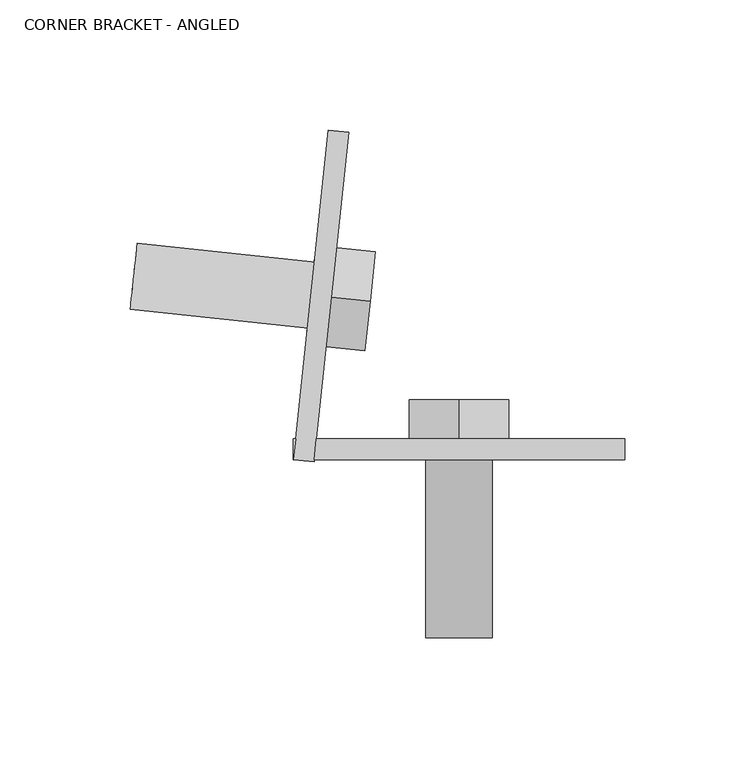
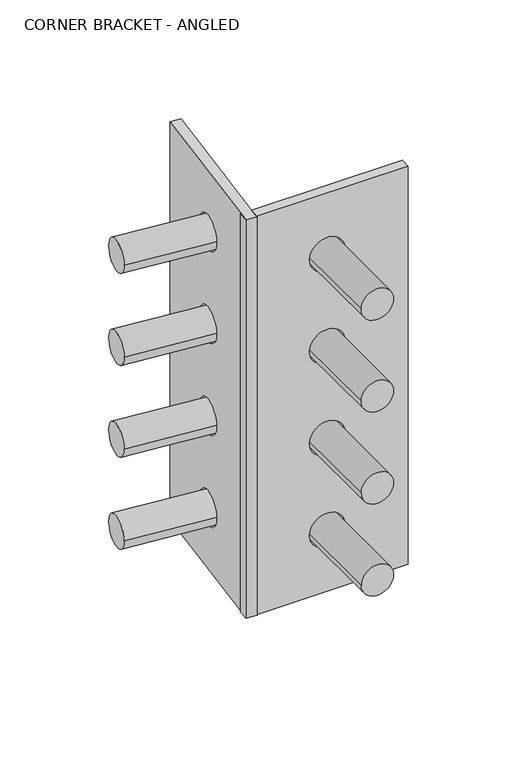
"""IFC4 building model written with IfcOpenShell, lengths in millimetres: fastener geometry, CORNER BRACKET - ANGLED."""

from ifc_helpers import new_model, si_unit, point, frame, frame_2d, origin, place, context, project, spatial, polyline, circle_curve, trimmed, segment, composite_curve, outline, extrude, faceted_brep, source, transform, mapped, element, save
from ifc_brep_helpers import plane_surface, revolved_surface, advanced_brep


def corner_bracket_angled_f47ab821(model_context):
    return source(origin(), model_context, "Body", "SolidModel", [
        advanced_brep(
        [(49.609375, 7.9375, 203.2), (77.390625, 7.9375, 203.2), (77.390625, 0.0, 203.2), (49.609375, 0.0, 203.2), (77.390625, 7.9375, 279.4), (49.609375, 7.9375, 279.4), (49.609375, 0.0, 279.4), (77.390625, 0.0, 279.4), (127.0, 0.0, 0.0), (127.0, 7.9375, 0.0), (127.0, 7.9375, 330.2), (127.0, 0.0, 330.2), (77.390625, 0.0, 127.0), (49.609375, 0.0, 127.0), (49.609375, 7.9375, 127.0), (77.390625, 7.9375, 127.0), (77.390625, 0.0, 50.8), (49.609375, 0.0, 50.8), (49.609375, 7.9375, 50.8), (77.390625, 7.9375, 50.8), (7.981222, 0.0, 330.2), (7.981222, 0.0, 0.0), (8.8154868, 7.9375, 0.0), (8.8154868, 7.9375, 330.2)],
        [
            (0, 1, circle_curve(frame((63.5, 7.9375, 203.2), z_axis=(0.0, 1.0, 0.0), x_axis=(-1.0000000000000002, 0.0, 0.0)), 13.890625)),
            (1, 2),
            (2, 3, circle_curve(frame((63.5, 0.0, 203.2), z_axis=(0.0, -1.0, 0.0), x_axis=(-1.0000000000000002, 0.0, 0.0)), 13.890625)),
            (3, 0),
            (4, 5, circle_curve(frame((63.5, 7.9375, 279.4), z_axis=(0.0, 1.0, 0.0), x_axis=(-1.0000000000000002, 0.0, 0.0)), 13.890625)),
            (5, 6),
            (6, 7, circle_curve(frame((63.5, 0.0, 279.4), z_axis=(0.0, -1.0, 0.0), x_axis=(-1.0000000000000002, 0.0, 0.0)), 13.890625)),
            (7, 4),
            (8, 9),
            (9, 10),
            (10, 11),
            (11, 8),
            (5, 4, circle_curve(frame((63.5, 7.9375, 279.4), z_axis=(0.0, 1.0, 0.0), x_axis=(-1.0000000000000002, 0.0, 0.0)), 13.890625)),
            (7, 6, circle_curve(frame((63.5, 0.0, 279.4), z_axis=(0.0, -1.0, 0.0), x_axis=(-1.0000000000000002, 0.0, 0.0)), 13.890625)),
            (12, 13, circle_curve(frame((63.5, 0.0, 127.0), z_axis=(0.0, -1.0, 0.0), x_axis=(-1.0000000000000002, 0.0, 0.0)), 13.890625)),
            (13, 14),
            (14, 15, circle_curve(frame((63.5, 7.9375, 127.0), z_axis=(0.0, 1.0, 0.0), x_axis=(-1.0000000000000002, 0.0, 0.0)), 13.890625)),
            (15, 12),
            (16, 17, circle_curve(frame((63.5, 0.0, 50.8), z_axis=(0.0, -1.0, 0.0), x_axis=(-1.0000000000000002, 0.0, 0.0)), 13.890625)),
            (17, 18),
            (18, 19, circle_curve(frame((63.5, 7.9375, 50.8), z_axis=(0.0, 1.0, 0.0), x_axis=(-1.0000000000000002, 0.0, 0.0)), 13.890625)),
            (19, 16),
            (11, 20),
            (20, 21),
            (21, 8),
            (2, 3, circle_curve(frame((63.5, 0.0, 203.2), z_axis=(0.0, 1.0, 0.0), x_axis=(-1.0000000000000002, 0.0, 0.0)), 13.890625)),
            (12, 13, circle_curve(frame((63.5, 0.0, 127.0), z_axis=(0.0, 1.0, 0.0), x_axis=(-1.0000000000000002, 0.0, 0.0)), 13.890625)),
            (16, 17, circle_curve(frame((63.5, 0.0, 50.8), z_axis=(0.0, 1.0, 0.0), x_axis=(-1.0000000000000002, 0.0, 0.0)), 13.890625)),
            (21, 22),
            (22, 9),
            (1, 0, circle_curve(frame((63.5, 7.9375, 203.2), z_axis=(0.0, 1.0, 0.0), x_axis=(-1.0000000000000002, 0.0, 0.0)), 13.890625)),
            (15, 14, circle_curve(frame((63.5, 7.9375, 127.0), z_axis=(0.0, 1.0, 0.0), x_axis=(-1.0000000000000002, 0.0, 0.0)), 13.890625)),
            (19, 18, circle_curve(frame((63.5, 7.9375, 50.8), z_axis=(0.0, 1.0, 0.0), x_axis=(-1.0000000000000002, 0.0, 0.0)), 13.890625)),
            (23, 22),
            (20, 23),
            (23, 10),
        ],
        [
            revolved_surface(polyline([(49.609375, 7.937500000000007, 203.2), (49.609375, 0.0, 203.2)]), (63.5, 0.0, 203.2), (0.0, 1.0000000000000004, 0.0)),
            revolved_surface(polyline([(49.609375, 7.937500000000007, 279.4), (49.609375, 0.0, 279.4)]), (63.5, 0.0, 279.4), (0.0, 1.0000000000000004, 0.0)),
            plane_surface(frame((127.0, 7.9375, 330.2), z_axis=(1.0, 0.0, 0.0), x_axis=(0.0, -1.0, 0.0))),
            revolved_surface(polyline([(49.609375, 7.937500000000007, 127.0), (49.609375, 0.0, 127.0)]), (63.5, 0.0, 127.0), (0.0, 1.0000000000000004, 0.0)),
            revolved_surface(polyline([(49.609375, 7.937500000000007, 50.8), (49.609375, 0.0, 50.8)]), (63.5, 0.0, 50.8), (0.0, 1.0000000000000004, 0.0)),
            plane_surface(frame((127.0, 0.0, 330.2), z_axis=(0.0, -1.0, 0.0), x_axis=(-1.0, 0.0, 0.0))),
            plane_surface(frame((127.0, 7.9375, 0.0), z_axis=(0.0, 0.0, -1.0), x_axis=(0.0, -1.0, 0.0))),
            plane_surface(frame((21.1691324, 125.474586, 330.2), z_axis=(-0.9945218953682732, 0.10452846326765532, 0.0), x_axis=(0.10452846326765532, 0.9945218953682732, 0.0))),
            plane_surface(frame((127.0, 7.9375, 330.2), z_axis=(0.0, 1.0, 0.0), x_axis=(1.0, 0.0, 0.0))),
            plane_surface(frame((0.0, 7.9375, 330.2), z_axis=(0.0, 0.0, 1.0), x_axis=(0.0, -1.0, 0.0))),
        ],
        [
            (0, [[1, 2, 3, 4]]),
            (1, [[5, 6, 7, 8]]),
            (2, [[9, 10, 11, 12]]),
            (1, [[13, -8, 14, -6]]),
            (3, [[15, 16, 17, 18]]),
            (4, [[19, 20, 21, 22]]),
            (5, [[-12, 23, 24, 25], [-7, -14], [26, -3], [-15, 27], [28, -19]]),
            (6, [[-9, -25, 29, 30]]),
            (0, [[31, -4, -26, -2]]),
            (3, [[32, -16, -27, -18]]),
            (4, [[33, -20, -28, -22]]),
            (7, [[34, -29, -24, 35]]),
            (8, [[-10, -30, -34, 36], [-5, -13], [-32, -17], [-31, -1], [-33, -21]]),
            (9, [[-11, -36, -35, -23]]),
        ],
    ),
        faceted_brep([(0.0, 7.9375, 0.0), (0.0, 7.9375, 330.2), (0.8342649, 7.9375, 330.2), (0.8342649, 7.9375, 0.0), (0.0, 0.0, 330.2), (0.0, 0.0, 0.0)], [[[0, 1, 2, 3]], [[1, 4, 2]], [[1, 0, 5, 4]], [[3, 2, 4, 5]], [[5, 0, 3]]]),
        extrude(outline(polyline([(290.3985226, 82.55), (301.3970453, 63.5), (290.3985226, 44.45), (268.4014774, 44.45), (257.4029547, 63.5), (268.4014774, 82.55), (290.3985226, 82.55)])), frame((0.0, 7.9375, 0.0), z_axis=(0.0, 1.0, 0.0), x_axis=(0.0, 0.0, 1.0)), (0.0, 0.0, 1.0), 14.9820312),
        extrude(outline(composite_curve([segment(trimmed(circle_curve(frame_2d((279.4, 63.5)), 12.7), [point((279.4, 76.2))], [point((279.4, 50.8))], False, "CARTESIAN"), True, "CONTINUOUS"), segment(trimmed(circle_curve(frame_2d((279.4, 63.5)), 12.7), [point((279.4, 50.8))], [point((279.4, 76.2))], False, "CARTESIAN"), True, "CONTINUOUS")], self_intersect=False)), frame((0.0, -68.2625, 0.0), z_axis=(0.0, 1.0, 0.0), x_axis=(0.0, 0.0, 1.0)), (0.0, 0.0, 1.0), 76.2),
        extrude(outline(polyline([(214.1985226, 82.55), (225.1970453, 63.5), (214.1985226, 44.45), (192.2014774, 44.45), (181.2029547, 63.5), (192.2014774, 82.55), (214.1985226, 82.55)])), frame((0.0, 7.9375, 0.0), z_axis=(0.0, 1.0, 0.0), x_axis=(0.0, 0.0, 1.0)), (0.0, 0.0, 1.0), 14.9820312),
        extrude(outline(composite_curve([segment(trimmed(circle_curve(frame_2d((203.2, 63.5)), 12.7), [point((203.2, 76.2))], [point((203.2, 50.8))], False, "CARTESIAN"), True, "CONTINUOUS"), segment(trimmed(circle_curve(frame_2d((203.2, 63.5)), 12.7), [point((203.2, 50.8))], [point((203.2, 76.2))], False, "CARTESIAN"), True, "CONTINUOUS")], self_intersect=False)), frame((0.0, -68.2625, 0.0), z_axis=(0.0, 1.0, 0.0), x_axis=(0.0, 0.0, 1.0)), (0.0, 0.0, 1.0), 76.2),
        extrude(outline(polyline([(290.3985226, 82.55), (301.3970453, 63.5), (290.3985226, 44.45), (268.4014774, 44.45), (257.4029547, 63.5), (268.4014774, 82.55), (290.3985226, 82.55)])), frame((0.0, 7.9375, 0.0), z_axis=(0.0, 1.0, 0.0), x_axis=(0.0, 0.0, 1.0)), (0.0, 0.0, 1.0), 14.9820312),
        extrude(outline(composite_curve([segment(trimmed(circle_curve(frame_2d((279.4, 63.5)), 12.7), [point((279.4, 76.2))], [point((279.4, 50.8))], False, "CARTESIAN"), True, "CONTINUOUS"), segment(trimmed(circle_curve(frame_2d((279.4, 63.5)), 12.7), [point((279.4, 50.8))], [point((279.4, 76.2))], False, "CARTESIAN"), True, "CONTINUOUS")], self_intersect=False)), frame((0.0, -68.2625, 0.0), z_axis=(0.0, 1.0, 0.0), x_axis=(0.0, 0.0, 1.0)), (0.0, 0.0, 1.0), 76.2),
        extrude(outline(polyline([(137.9985226, 82.55), (148.9970453, 63.5), (137.9985226, 44.45), (116.0014774, 44.45), (105.0029547, 63.5), (116.0014774, 82.55), (137.9985226, 82.55)])), frame((0.0, 7.9375, 0.0), z_axis=(0.0, 1.0, 0.0), x_axis=(0.0, 0.0, 1.0)), (0.0, 0.0, 1.0), 14.9820312),
        extrude(outline(composite_curve([segment(trimmed(circle_curve(frame_2d((127.0, 63.5)), 12.7), [point((127.0, 76.2))], [point((127.0, 50.8))], False, "CARTESIAN"), True, "CONTINUOUS"), segment(trimmed(circle_curve(frame_2d((127.0, 63.5)), 12.7), [point((127.0, 50.8))], [point((127.0, 76.2))], False, "CARTESIAN"), True, "CONTINUOUS")], self_intersect=False)), frame((0.0, -68.2625, 0.0), z_axis=(0.0, 1.0, 0.0), x_axis=(0.0, 0.0, 1.0)), (0.0, 0.0, 1.0), 76.2),
        extrude(outline(polyline([(61.7985226, 82.55), (72.7970453, 63.5), (61.7985226, 44.45), (39.8014774, 44.45), (28.8029547, 63.5), (39.8014774, 82.55), (61.7985226, 82.55)])), frame((0.0, 7.9375, 0.0), z_axis=(0.0, 1.0, 0.0), x_axis=(0.0, 0.0, 1.0)), (0.0, 0.0, 1.0), 14.9820312),
        extrude(outline(composite_curve([segment(trimmed(circle_curve(frame_2d((50.8, 63.5)), 12.7), [point((50.8, 76.2))], [point((50.8, 50.8))], False, "CARTESIAN"), True, "CONTINUOUS"), segment(trimmed(circle_curve(frame_2d((50.8, 63.5)), 12.7), [point((50.8, 50.8))], [point((50.8, 76.2))], False, "CARTESIAN"), True, "CONTINUOUS")], self_intersect=False)), frame((0.0, -68.2625, 0.0), z_axis=(0.0, 1.0, 0.0), x_axis=(0.0, 0.0, 1.0)), (0.0, 0.0, 1.0), 76.2),
        advanced_brep(
        [(15.9835406, 76.1369764, 203.2), (13.0796093, 48.507915, 203.2), (5.1855917, 49.3376097, 203.2), (8.0895231, 76.9666711, 203.2), (8.0895231, 76.9666711, 279.4), (5.1855917, 49.3376097, 279.4), (13.0796093, 48.507915, 279.4), (15.9835406, 76.1369764, 279.4), (21.1691324, 125.474586, 0.0), (13.2751148, 126.3042807, 0.0), (13.2751148, 126.3042807, 330.2), (21.1691324, 125.474586, 330.2), (15.9835406, 76.1369764, 127.0), (13.0796093, 48.507915, 127.0), (5.1855917, 49.3376097, 127.0), (8.0895231, 76.9666711, 127.0), (15.9835406, 76.1369764, 50.8), (13.0796093, 48.507915, 50.8), (5.1855917, 49.3376097, 50.8), (8.0895231, 76.9666711, 50.8), (7.8940175, -0.8296947, 330.2), (7.8940175, -0.8296947, 0.0), (7.981222, 0.0, 0.0), (8.8154868, 7.9375, 0.0), (8.8154868, 7.9375, 330.2), (7.981222, 0.0, 330.2), (0.0, 0.0, 330.2), (0.8342649, 7.9375, 330.2), (0.8342649, 7.9375, 0.0), (0.0, 0.0, 0.0)],
        [
            (0, 1, circle_curve(frame((14.531575, 62.3224457, 203.2), z_axis=(0.9945218953682732, -0.10452846326765532, 0.0), x_axis=(-0.10452846326765532, -0.9945218953682732, 0.0)), 13.890625)),
            (1, 2),
            (2, 3, circle_curve(frame((6.6375574, 63.1521404, 203.2), z_axis=(-0.9945218953682732, 0.10452846326765532, 0.0), x_axis=(-0.10452846326765532, -0.9945218953682732, 0.0)), 13.890625)),
            (3, 0),
            (4, 5, circle_curve(frame((6.6375574, 63.1521404, 279.4), z_axis=(-0.9945218953682732, 0.10452846326765532, 0.0), x_axis=(-0.10452846326765532, -0.9945218953682732, 0.0)), 13.890625)),
            (5, 6),
            (6, 7, circle_curve(frame((14.531575, 62.3224457, 279.4), z_axis=(0.9945218953682732, -0.10452846326765532, 0.0), x_axis=(-0.10452846326765532, -0.9945218953682732, 0.0)), 13.890625)),
            (7, 4),
            (8, 9),
            (9, 10),
            (10, 11),
            (11, 8),
            (7, 6, circle_curve(frame((14.531575, 62.3224457, 279.4), z_axis=(0.9945218953682732, -0.10452846326765532, 0.0), x_axis=(-0.10452846326765532, -0.9945218953682732, 0.0)), 13.890625)),
            (5, 4, circle_curve(frame((6.6375574, 63.1521404, 279.4), z_axis=(-0.9945218953682732, 0.10452846326765532, 0.0), x_axis=(-0.10452846326765532, -0.9945218953682732, 0.0)), 13.890625)),
            (12, 13, circle_curve(frame((14.531575, 62.3224457, 127.0), z_axis=(0.9945218953682732, -0.10452846326765532, 0.0), x_axis=(-0.10452846326765532, -0.9945218953682732, 0.0)), 13.890625)),
            (13, 14),
            (14, 15, circle_curve(frame((6.6375574, 63.1521404, 127.0), z_axis=(-0.9945218953682732, 0.10452846326765532, 0.0), x_axis=(-0.10452846326765532, -0.9945218953682732, 0.0)), 13.890625)),
            (15, 12),
            (16, 17, circle_curve(frame((14.531575, 62.3224457, 50.8), z_axis=(0.9945218953682732, -0.10452846326765532, 0.0), x_axis=(-0.10452846326765532, -0.9945218953682732, 0.0)), 13.890625)),
            (17, 18),
            (18, 19, circle_curve(frame((6.6375574, 63.1521404, 50.8), z_axis=(-0.9945218953682732, 0.10452846326765532, 0.0), x_axis=(-0.10452846326765532, -0.9945218953682732, 0.0)), 13.890625)),
            (19, 16),
            (20, 21),
            (21, 22),
            (22, 23),
            (23, 8),
            (11, 24),
            (24, 25),
            (25, 20),
            (0, 1, circle_curve(frame((14.531575, 62.3224457, 203.2), z_axis=(-0.9945218953682732, 0.10452846326765532, 0.0), x_axis=(-0.10452846326765532, -0.9945218953682732, 0.0)), 13.890625)),
            (16, 17, circle_curve(frame((14.531575, 62.3224457, 50.8), z_axis=(-0.9945218953682732, 0.10452846326765532, 0.0), x_axis=(-0.10452846326765532, -0.9945218953682732, 0.0)), 13.890625)),
            (12, 13, circle_curve(frame((14.531575, 62.3224457, 127.0), z_axis=(-0.9945218953682732, 0.10452846326765532, 0.0), x_axis=(-0.10452846326765532, -0.9945218953682732, 0.0)), 13.890625)),
            (26, 27),
            (27, 10),
            (9, 28),
            (28, 29),
            (29, 26),
            (2, 3, circle_curve(frame((6.6375574, 63.1521404, 203.2), z_axis=(0.9945218953682732, -0.10452846326765532, 0.0), x_axis=(-0.10452846326765532, -0.9945218953682732, 0.0)), 13.890625)),
            (18, 19, circle_curve(frame((6.6375574, 63.1521404, 50.8), z_axis=(0.9945218953682732, -0.10452846326765532, 0.0), x_axis=(-0.10452846326765532, -0.9945218953682732, 0.0)), 13.890625)),
            (14, 15, circle_curve(frame((6.6375574, 63.1521404, 127.0), z_axis=(0.9945218953682732, -0.10452846326765532, 0.0), x_axis=(-0.10452846326765532, -0.9945218953682732, 0.0)), 13.890625)),
            (26, 20),
            (21, 29),
        ],
        [
            revolved_surface(polyline([(13.079609316687709, 48.507915013942764, 203.2), (5.185591699866783, 49.33760969873252, 203.2)]), (6.6375574, 63.1521404, 203.2), (0.9945218953682732, -0.10452846326765532, 0.0)),
            revolved_surface(polyline([(13.079609316687709, 48.507915013942764, 279.4), (5.185591699866783, 49.33760969873252, 279.4)]), (6.6375574, 63.1521404, 279.4), (0.9945218953682732, -0.10452846326765532, 0.0)),
            plane_surface(frame((21.1691324, 125.474586, 330.2), z_axis=(0.10452846326765532, 0.9945218953682732, 0.0), x_axis=(-0.9945218953682732, 0.10452846326765532, 0.0))),
            revolved_surface(polyline([(13.079609316687709, 48.507915013942764, 127.0), (5.185591699866783, 49.33760969873252, 127.0)]), (6.6375574, 63.1521404, 127.0), (0.9945218953682732, -0.10452846326765532, 0.0)),
            revolved_surface(polyline([(13.079609316687709, 48.507915013942764, 50.8), (5.185591699866783, 49.33760969873252, 50.8)]), (6.6375574, 63.1521404, 50.8), (0.9945218953682732, -0.10452846326765532, 0.0)),
            plane_surface(frame((21.1691324, 125.474586, 330.2), z_axis=(0.9945218953682732, -0.10452846326765532, 0.0), x_axis=(0.10452846326765532, 0.9945218953682732, 0.0))),
            plane_surface(frame((13.2751148, 126.3042807, 330.2), z_axis=(-0.9945218953682732, 0.10452846326765532, 0.0), x_axis=(-0.10452846326765532, -0.9945218953682732, 0.0))),
            plane_surface(frame((7.8940175, -0.8296947, 330.2), z_axis=(0.0, 0.0, 1.0), x_axis=(-0.9945218953682732, 0.10452846326765532, 0.0))),
            plane_surface(frame((21.1691324, 125.474586, 0.0), z_axis=(0.0, 0.0, -1.0), x_axis=(-0.9945218953682732, 0.10452846326765532, 0.0))),
            plane_surface(frame((7.8940175, -0.8296947, 0.0), z_axis=(-0.10452846326765532, -0.9945218953682732, 0.0), x_axis=(-0.9945218953682732, 0.10452846326765532, 0.0))),
        ],
        [
            (0, [[1, 2, 3, 4]]),
            (1, [[5, 6, 7, 8]]),
            (2, [[9, 10, 11, 12]]),
            (1, [[13, -6, 14, -8]]),
            (3, [[15, 16, 17, 18]]),
            (4, [[19, 20, 21, 22]]),
            (5, [[23, 24, 25, 26, -12, 27, 28, 29], [-13, -7], [-1, 30], [-19, 31], [-15, 32]]),
            (6, [[33, 34, -10, 35, 36, 37], [-14, -5], [-3, 38], [-21, 39], [-17, 40]]),
            (7, [[-11, -34, -33, 41, -29, -28, -27]]),
            (8, [[42, -36, -35, -9, -26, -25, -24]]),
            (9, [[-41, -37, -42, -23]]),
            (0, [[-38, -2, -30, -4]]),
            (3, [[-40, -16, -32, -18]]),
            (4, [[-39, -20, -31, -22]]),
        ],
    ),
        extrude(outline(polyline([(0.0, 0.0), (-10.9985227, 19.05), (0.0, 38.1), (21.9970452, 38.1), (32.9955679, 19.05), (21.9970452, 0.0), (0.0, 0.0)])), frame((31.4228003, 79.7020391, 290.3985226), z_axis=(-0.9945218953682732, 0.10452846326765532, 0.0), x_axis=(0.0, 0.0, -1.0)), (0.0, 0.0, 1.0), 14.9820312),
        extrude(outline(composite_curve([segment(trimmed(circle_curve(frame_2d((0.0, 12.7)), 12.7), [point((0.0, 25.4))], [point((0.0, 0.0))], False, "CARTESIAN"), True, "CONTINUOUS"), segment(trimmed(circle_curve(frame_2d((0.0, 12.7)), 12.7), [point((0.0, 0.0))], [point((0.0, 25.4))], False, "CARTESIAN"), True, "CONTINUOUS")], self_intersect=False)), frame((13.2040635, 49.6920176, 279.4), z_axis=(-0.9945218953682732, 0.10452846326765532, 0.0), x_axis=(0.0, 0.0, 1.0)), (0.0, 0.0, 1.0), 76.2),
        extrude(outline(polyline([(0.0, 0.0), (-10.9985227, 19.05), (0.0, 38.1), (21.9970452, 38.1), (32.9955679, 19.05), (21.9970452, 0.0), (0.0, 0.0)])), frame((31.4228003, 79.7020391, 214.1985226), z_axis=(-0.9945218953682732, 0.10452846326765532, 0.0), x_axis=(0.0, 0.0, -1.0)), (0.0, 0.0, 1.0), 14.9820312),
        extrude(outline(composite_curve([segment(trimmed(circle_curve(frame_2d((0.0, 12.7)), 12.7), [point((0.0, 25.4))], [point((0.0, 0.0))], False, "CARTESIAN"), True, "CONTINUOUS"), segment(trimmed(circle_curve(frame_2d((0.0, 12.7)), 12.7), [point((0.0, 0.0))], [point((0.0, 25.4))], False, "CARTESIAN"), True, "CONTINUOUS")], self_intersect=False)), frame((13.2040635, 49.6920176, 203.2), z_axis=(-0.9945218953682732, 0.10452846326765532, 0.0), x_axis=(0.0, 0.0, 1.0)), (0.0, 0.0, 1.0), 76.2),
        extrude(outline(polyline([(0.0, 0.0), (-10.9985227, 19.05), (0.0, 38.1), (21.9970452, 38.1), (32.9955679, 19.05), (21.9970452, 0.0), (0.0, 0.0)])), frame((31.4228003, 79.7020391, 290.3985226), z_axis=(-0.9945218953682732, 0.10452846326765532, 0.0), x_axis=(0.0, 0.0, -1.0)), (0.0, 0.0, 1.0), 14.9820312),
        extrude(outline(composite_curve([segment(trimmed(circle_curve(frame_2d((0.0, 12.7)), 12.7), [point((0.0, 25.4))], [point((0.0, 0.0))], False, "CARTESIAN"), True, "CONTINUOUS"), segment(trimmed(circle_curve(frame_2d((0.0, 12.7)), 12.7), [point((0.0, 0.0))], [point((0.0, 25.4))], False, "CARTESIAN"), True, "CONTINUOUS")], self_intersect=False)), frame((13.2040635, 49.6920176, 279.4), z_axis=(-0.9945218953682732, 0.10452846326765532, 0.0), x_axis=(0.0, 0.0, 1.0)), (0.0, 0.0, 1.0), 76.2),
        extrude(outline(polyline([(0.0, 0.0), (-10.9985227, 19.05), (0.0, 38.1), (21.9970452, 38.1), (32.9955679, 19.05), (21.9970452, 0.0), (0.0, 0.0)])), frame((31.4228003, 79.7020391, 137.9985226), z_axis=(-0.9945218953682732, 0.10452846326765532, 0.0), x_axis=(0.0, 0.0, -1.0)), (0.0, 0.0, 1.0), 14.9820312),
        extrude(outline(composite_curve([segment(trimmed(circle_curve(frame_2d((0.0, 12.7)), 12.7), [point((0.0, 25.4))], [point((0.0, 0.0))], False, "CARTESIAN"), True, "CONTINUOUS"), segment(trimmed(circle_curve(frame_2d((0.0, 12.7)), 12.7), [point((0.0, 0.0))], [point((0.0, 25.4))], False, "CARTESIAN"), True, "CONTINUOUS")], self_intersect=False)), frame((13.2040635, 49.6920176, 127.0), z_axis=(-0.9945218953682732, 0.10452846326765532, 0.0), x_axis=(0.0, 0.0, 1.0)), (0.0, 0.0, 1.0), 76.2),
        extrude(outline(polyline([(0.0, 0.0), (-10.9985227, 19.05), (0.0, 38.1), (21.9970452, 38.1), (32.9955679, 19.05), (21.9970452, 0.0), (0.0, 0.0)])), frame((31.4228003, 79.7020391, 61.7985226), z_axis=(-0.9945218953682732, 0.10452846326765532, 0.0), x_axis=(0.0, 0.0, -1.0)), (0.0, 0.0, 1.0), 14.9820312),
        extrude(outline(composite_curve([segment(trimmed(circle_curve(frame_2d((0.0, 12.7)), 12.7), [point((0.0, 25.4))], [point((0.0, 0.0))], False, "CARTESIAN"), True, "CONTINUOUS"), segment(trimmed(circle_curve(frame_2d((0.0, 12.7)), 12.7), [point((0.0, 0.0))], [point((0.0, 25.4))], False, "CARTESIAN"), True, "CONTINUOUS")], self_intersect=False)), frame((13.2040635, 49.6920176, 50.8), z_axis=(-0.9945218953682732, 0.10452846326765532, 0.0), x_axis=(0.0, 0.0, 1.0)), (0.0, 0.0, 1.0), 76.2),
    ])


if __name__ == "__main__":
    model = new_model("IFC4")
    model_context = context("Model", 3, world=origin())
    ifc_project = project(units=[si_unit("LENGTHUNIT", "METRE", prefix="MILLI")], contexts=[model_context])
    site = spatial("IfcSite", under=ifc_project)
    building = spatial("IfcBuilding", under=site)
    placement = place(None, origin())
    corner_bracket_angled_shape = corner_bracket_angled_f47ab821(model_context)
    element("IfcFastener", 1, ObjectType="CORNER BRACKET - ANGLED : CUSTOM - L5\"x5\"x5/16\"x13\" (BENT ANGLE - 84°) - HDG", at=placement, inside=building, context=model_context, shape_type="MappedRepresentation", body=[
        mapped(corner_bracket_angled_shape, transform((0.0, 0.0, 0.0), x_axis=(1.0, 0.0, 0.0), y_axis=(0.0, 1.0, 0.0), z_axis=(0.0, 0.0, 1.0))),
    ])
    save(model, "model.ifc")

# Revit data of these elements
# Type "CORNER BRACKET - ANGLED : CUSTOM - L5\"x5\"x5/16\"x13\" (BENT ANGLE - 84°) - HDG"
#   URL = "https://www.strongtie.com/classiccollection_architecturalproductsgroup/hlpc-hlgpc_productgroup_wcc/p/hlpc.hlgpc"
#   Default Elevation = 4' - 0"
#   Angle = 84.00°
#   Leg Two = element 1900782
#   Leg One = element 1900782
#   URL = ""
# Element 1 (IfcFastener, "CORNER BRACKET - ANGLED : CUSTOM - L5\"x5\"x5/16\"x13\" (BENT ANGLE - 84°) - HDG")
#   Materials on its faces: "1\" GALV. LAG BOLT (LENGTH = 1/2\" SHY OF GLULAM DEPTH) -  (GALV. THRU BOLT IF PLATE ON OPP. SIDE OF STRUCT MEMBER)", "L5\"x5\"x5/16\" STEEL ANGLE (HDG AFTER FABRICATION)"
# Materials
#   "1\" GALV. LAG BOLT (LENGTH = 1/2\" SHY OF GLULAM DEPTH) -  (GALV. THRU BOLT IF PLATE ON OPP. SIDE OF STRUCT MEMBER)": class "Generic", colour RGB 120 120 120, transparency 0, Cost = 0
#   "L5\"x5\"x5/16\" STEEL ANGLE (HDG AFTER FABRICATION)": class "Generic", colour RGB 232 232 232, transparency 0, Cost = 0
